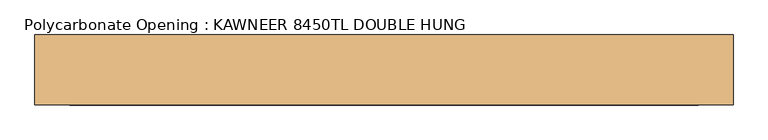
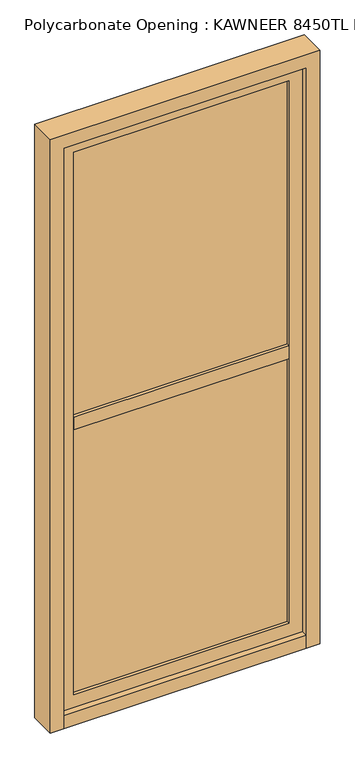
"""IFC4 building model written with IfcOpenShell, lengths in millimetres: door geometry, Polycarbonate Opening : KAWNEER 8450TL DOUBLE HUNG."""

from ifc_helpers import new_model, si_unit, frame, origin, origin_with_axes, place, context, project, spatial, polyline, outline, extrude, source, transform, mapped, element, save


def polycarbonate_opening_kawneer_8450tl_double_hung_5184030a(model_context):
    return source(origin(), model_context, "Body", "SweptSolid", [
        extrude(outline(polyline([(457.2, 0.0), (-457.2, 0.0), (-457.2, 25.4), (457.2, 25.4), (457.2, 0.0)])), frame((0.0, 0.0, 50.8), z_axis=(0.0, 0.0, 1.0), x_axis=(1.0, 0.0, 0.0)), (0.0, 0.0, 1.0), 2260.6),
        extrude(outline(polyline([(2311.4, -457.2), (0.0, -457.2), (0.0, 457.2), (2311.4, 457.2), (2311.4, -457.2)]), holes=[polyline([(101.6, 406.4), (101.6, -406.4), (2260.6, -406.4), (2260.6, 406.4), (101.6, 406.4)])]), frame((0.0, -12.7, 0.0), z_axis=(0.0, 1.0, 0.0), x_axis=(0.0, 0.0, 1.0)), (0.0, 0.0, 1.0), 50.8),
        extrude(outline(polyline([(2362.2, 508.0), (2362.2, -508.0), (0.0, -508.0), (0.0, -457.2), (2311.4, -457.2), (2311.4, 457.2), (0.0, 457.2), (0.0, 508.0), (2362.2, 508.0)])), frame((0.0, -38.1, 0.0), z_axis=(0.0, 1.0, 0.0), x_axis=(0.0, 0.0, 1.0)), (0.0, 0.0, 1.0), 101.6),
        extrude(outline(polyline([(406.4, -12.7), (-406.4, -12.7), (-406.4, 38.1), (406.4, 38.1), (406.4, -12.7)])), frame((0.0, 0.0, 1155.7), z_axis=(0.0, 0.0, 1.0), x_axis=(1.0, 0.0, 0.0)), (0.0, 0.0, 1.0), 50.8),
        extrude(outline(polyline([(457.2, -38.1), (-457.2, -38.1), (-457.2, 63.5), (457.2, 63.5), (457.2, -38.1)])), origin_with_axes(), (0.0, 0.0, 1.0), 50.8),
    ])


if __name__ == "__main__":
    model = new_model("IFC4")
    model_context = context("Model", 3, world=origin())
    ifc_project = project(units=[si_unit("LENGTHUNIT", "METRE", prefix="MILLI")], contexts=[model_context])
    site = spatial("IfcSite", under=ifc_project)
    building = spatial("IfcBuilding", under=site)
    placement = place(None, origin())
    polycarbonate_opening_kawneer_8450tl_double_hung_shape = polycarbonate_opening_kawneer_8450tl_double_hung_5184030a(model_context)
    element("IfcDoor", 1, ObjectType="Polycarbonate Opening : KAWNEER 8450TL DOUBLE HUNG", at=placement, inside=building, context=model_context, shape_type="MappedRepresentation", body=[
        mapped(polycarbonate_opening_kawneer_8450tl_double_hung_shape, transform((0.0, 0.0, 0.0), x_axis=(1.0, 0.0, 0.0), y_axis=(0.0, 1.0, 0.0), z_axis=(0.0, 0.0, 1.0))),
    ])
    save(model, "model.ifc")

# Revit data of these elements
# Type "Polycarbonate Opening : KAWNEER 8450TL DOUBLE HUNG"
#   Type Mark = "59"
#   OD_DS_Door_Material = "ALUM./GLAZING"
#   OD_DS_Door_Type = "STOREFRONT - SINGLE HUNG WINDOW"
#   OD_DS_Lockset = "-"
#   Analytic Construction = "<None>"
#   offset [instance default] = 0' - 2"
#   Stile = 0' - 2"
#   Mullion Width = 0' - 2"
#   Mullion Depth = 0' - 4"
#   Opening Size [instance default] = 5' - 1.50212"
#   Door Width [instance default] = 5' - 1.50212"
#   Window ON/OFF = no
#   Door On/Off = yes
#   Mullion Material = KAWNEER 8450TL DOUBLE HUNG (CLEAR ANODIZED ALUM) - TEMPERED INSULATED GLAZING (CARDINAL GLASS LoĒ²-240\nOR EQUIVALENT)
#   Glass Material = TEMPERED INSULATED GLAZING (CARDINAL GLASS LoĒ²-240\nOR EQUIVALENT)
#   Door Material = KAWNEER 8450TL DOUBLE HUNG (CLEAR ANODIZED ALUM) - TEMPERED INSULATED GLAZING (CARDINAL GLASS LoĒ²-240\nOR EQUIVALENT)
# Element 1 (IfcDoor, "Polycarbonate Opening : KAWNEER 8450TL DOUBLE HUNG")
#   offset = 0' - 0 1/2"
#   Materials on its faces: "KAWNEER 8450TL DOUBLE HUNG (CLEAR ANODIZED ALUM) - TEMPERED INSULATED GLAZING (CARDINAL GLASS LoĒ²-240\nOR EQUIVALENT)", "TEMPERED INSULATED GLAZING (CARDINAL GLASS LoĒ²-240\nOR EQUIVALENT)"
# Materials
#   "KAWNEER 8450TL DOUBLE HUNG (CLEAR ANODIZED ALUM) - TEMPERED INSULATED GLAZING (CARDINAL GLASS LoĒ²-240\nOR EQUIVALENT)": class "Metal", colour RGB 244 244 244, transparency 0, Description = "Aluminum 6061", Cost = 0
#   "TEMPERED INSULATED GLAZING (CARDINAL GLASS LoĒ²-240\nOR EQUIVALENT)": class "Glass", colour RGB 196 205 210, transparency 0.85, Description = "Soda Lime Glass", Cost = 0
